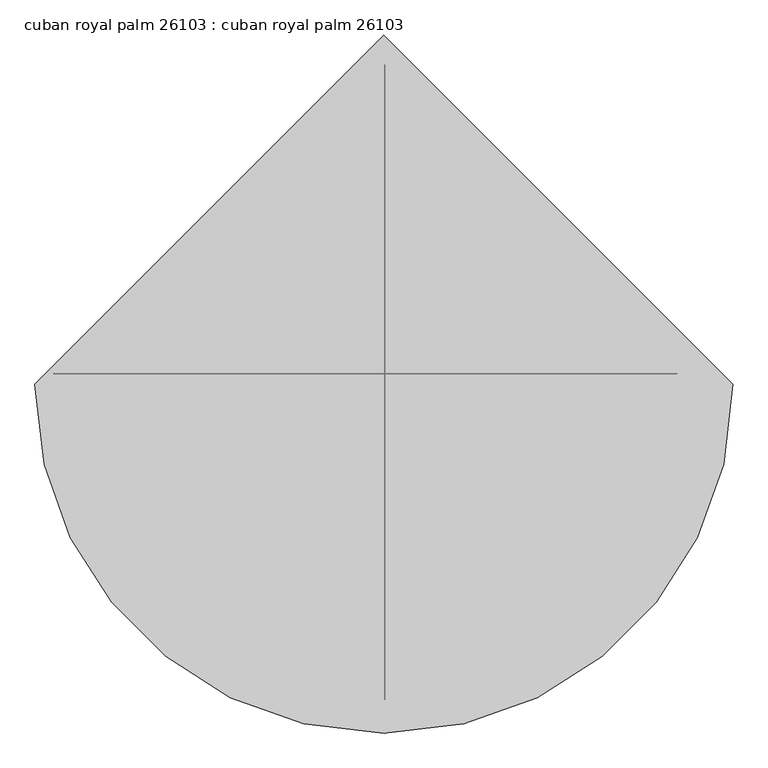
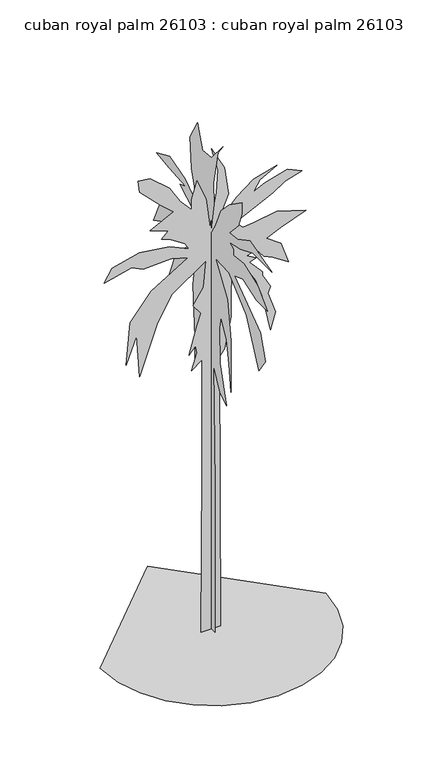
"""IFC4 building model written with IfcOpenShell, lengths in millimetres: proxy geometry, cuban royal palm 26103 : cuban royal palm 26103."""

from ifc_helpers import new_model, si_unit, origin, place, context, project, spatial, triangles, source, transform, mapped, element, save


def cuban_royal_palm_26103_cuban_royal_palm_26103_6f0ceb55(model_context):
    return source(origin(), model_context, "Body", "Tessellation", [
        triangles([(-54.3826135, -0.017491, 0.0009437), (-150.0419681, -0.0174994, 0.0009479), (-130.9099418, -0.0179382, 2494.6483109), (-130.9096875, -0.0182426, 4197.3711227), (-283.9640988, -0.0182154, 4082.5885941), (-207.4377743, -0.0182632, 4331.3053894), (-226.5690375, -0.0182829, 4446.0876274), (-322.2291687, -0.0182582, 4331.3053894), (-207.4375199, -0.0183385, 4752.2081863), (-150.0417137, -0.0183718, 4924.3947693), (-264.8328356, -0.0183942, 5077.4551941), (-111.778179, -0.0184419, 5307.0196701), (-73.5143854, -0.0185154, 5708.7968903), (-570.9431663, -0.0184321, 5364.4237244), (-781.3921303, -0.0183579, 5000.9249817), (-1049.2399527, -0.0182128, 4254.775177), (-1087.5024427, -0.0183274, 4905.2686111), (-1240.5575626, -0.0182489, 4503.4916817), (-1183.1638275, -0.0183643, 5134.8336685), (-877.0535151, -0.0184461, 5517.4841492), (-341.3604137, -0.0185277, 5842.7305756), (-590.0744476, -0.0185305, 5919.260788), (-991.8436014, -0.0185095, 5900.10905), (-1164.030039, -0.0185156, 5976.6392624), (-1565.7991928, -0.018481, 5880.9828918), (-1451.0091064, -0.0185202, 6072.2956329), (-1049.2399527, -0.0185549, 6167.9775833), (-609.2056927, -0.0185639, 6110.5735291), (-322.2291687, -0.0185524, 5976.6392624), (-379.6254836, -0.018567, 6072.2956329), (-609.2056927, -0.0185844, 6225.3560577), (-723.9983225, -0.0185862, 6263.6339539), (-628.3394812, -0.0186075, 6359.2903244), (-896.1847601, -0.0186129, 6454.9461136), (-551.8119212, -0.0186587, 6627.1326965), (-743.1295675, -0.0186811, 6799.3192795), (-1049.2399527, -0.0187225, 7105.4395477), (-1068.3711977, -0.0187524, 7277.6261307), (-896.1847601, -0.0187566, 7258.4743927), (-609.2056927, -0.0187246, 7009.7581787), (-456.1505364, -0.0186868, 6761.0413834), (-283.9640988, -0.0186602, 6569.7286423), (-283.9640988, -0.0186875, 6722.7890671), (-207.4375199, -0.0187388, 6990.6320206), (-73.5143854, -0.0186865, 6665.3850128), (-16.1188494, -0.0186069, 6206.2298996), (79.5405301, -0.0187, 6703.6629089), (98.6725473, -0.0187624, 7048.0354935), (3.0131737, -0.0188232, 7411.5348175), (194.3319064, -0.0187666, 7048.0354935), (251.7277126, -0.0186938, 6627.1326965), (79.5405301, -0.018611, 6206.2298996), (366.5190888, -0.0186818, 6531.476326), (615.2330864, -0.0187268, 6722.7890671), (959.6059616, -0.018759, 6818.4454376), (710.8919277, -0.0187242, 6684.5367508), (615.2330864, -0.0186926, 6531.476326), (787.419524, -0.0187138, 6608.0065384), (1112.6611542, -0.0187452, 6703.6629089), (1323.1125526, -0.0187373, 6608.0065384), (1074.3985914, -0.0187127, 6531.476326), (902.2121538, -0.0186847, 6416.6687988), (347.3878438, -0.0186125, 6148.8258453), (462.1779302, -0.018597, 6034.0433167), (615.2330864, -0.0186071, 6053.1694748), (959.6059616, -0.0186324, 6110.5735291), (1380.5089039, -0.0186269, 5976.6392624), (1017.0023129, -0.018587, 5842.7305756), (806.550769, -0.0185607, 5747.074205), (1017.0023129, -0.0185426, 5594.0143616), (1131.7923992, -0.0184894, 5268.7673538), (902.2121538, -0.0185068, 5421.8277786), (768.288279, -0.0185112, 5479.2062531), (615.2330864, -0.0185387, 5670.544574), (615.2330864, -0.0185284, 5613.1405197), (519.5742451, -0.0185174, 5574.8882034), (653.4956491, -0.0185096, 5498.357991), (557.8367715, -0.0184985, 5460.0800949), (749.1570339, -0.0184693, 5249.6411957), (749.1570339, -0.018459, 5192.2371414), (863.9471203, -0.0184264, 4981.7988235), (825.6846302, -0.0184076, 4886.142453), (940.4747166, -0.0183545, 4560.8957359), (863.9471203, -0.0183067, 4312.1792313), (749.1570339, -0.0184009, 4866.990715), (653.4956491, -0.018448, 5153.9848251), (481.3092115, -0.0184918, 5440.9539368), (309.1227739, -0.0184979, 5517.4841492), (289.9915107, -0.0184287, 5134.8336685), (289.9915107, -0.0183534, 4713.9558701), (194.3319064, -0.0182671, 4254.775177), (117.8043192, -0.0182467, 4159.1188065), (136.9360911, -0.0175052, 0.0009354), (-0.003708, 89.5986644, 0.000495), (-0.0037084, 163.6334895, 0.0005082), (-0.003708, 163.6334895, 1826.7789024), (-0.003706, 145.1250443, 4288.4300995), (-0.0037076, 219.1593699, 4177.3813545), (-0.0037057, 404.2456741, 3788.6856033), (-0.0037071, 404.2456741, 4251.4224747), (-0.0037068, 459.7725537, 5028.7883972), (-0.0037083, 385.7367022, 5565.5410995), (-0.0037091, 533.8058619, 5398.9425476), (-0.0037068, 792.9287807, 4862.190136), (-0.0037064, 1089.0671001, 4492.0362762), (-0.0037084, 1311.1695316, 4140.3737297), (-0.0037071, 1052.0491562, 4843.6988228), (-0.0037074, 885.4710245, 5250.8858871), (-0.0037074, 515.2968899, 5621.065036), (-0.003709, 681.8750216, 5584.0318314), (-0.0037073, 903.9799965, 5565.5410995), (-0.0037076, 1107.5760721, 5602.5487244), (-0.0037076, 1459.2413074, 5417.4588593), (-0.0037087, 1274.1542038, 5824.6462143), (-0.0037067, 1070.5581282, 5824.6462143), (-0.0037071, 996.5223129, 6139.3008453), (-0.0037076, 644.859621, 6065.2600159), (-0.0037089, 422.7546461, 6176.3084702), (-0.0037091, 792.9287807, 6379.9146469), (-0.0037059, 644.859621, 6435.4391647), (-0.0037081, 1052.0491562, 6472.4467896), (-0.0037064, 1385.2054195, 6509.4799942), (-0.0037073, 1052.0491562, 6657.5366547), (-0.0037075, 663.368593, 6546.487619), (-0.0037092, 348.7187945, 6324.3907104), (-0.003707, 496.7904977, 6805.6183136), (-0.0037068, 533.8058619, 7268.3296051), (-0.0037076, 348.7187945, 7601.4755493), (-0.0037068, 311.703394, 7490.427095), (-0.0037069, 219.1593699, 7249.8132935), (-0.0037086, -2.9445681, 7268.3296051), (-0.0037062, -299.0821622, 7619.9924423), (-0.0037078, -169.5227376, 7453.4194702), (-0.0037084, -58.4704863, 6916.6673492), (-0.0037085, -76.9791948, 6602.0121368), (-0.003709, 15.5640629, 6083.7763275), (-0.0037058, -113.9968663, 6287.3575058), (-0.0037085, -243.5573174, 6602.0121368), (-0.0037085, -465.6602757, 6824.1096268), (-0.003709, -780.3075308, 7046.2321152), (-0.003709, -780.3075308, 6879.6341446), (-0.0037083, -687.765287, 6639.0453415), (-0.0037091, -465.6602757, 6398.4315399), (-0.0037063, -669.256315, 6416.9228531), (-0.0037092, -983.9036064, 6583.4958252), (-0.0037074, -1539.164772, 6435.4391647), (-0.0037081, -1057.9394217, 6435.4391647), (-0.0037072, -743.2921303, 6305.8738174), (-0.0037083, -465.6602757, 6250.3492996), (-0.0037076, -558.2050993, 6194.8253632), (-0.003708, -558.2050993, 6102.2932205), (-0.0037077, -835.8344467, 6139.3008453), (-0.0037071, -1187.4996094, 6009.735498), (-0.0037064, -1428.1110855, 5769.1216965), (-0.0037087, -1150.4816654, 5769.1216965), (-0.0037066, -798.8165028, 5880.1701508), (-0.0037081, -595.2230069, 5806.1549011), (-0.0037069, -1243.0264526, 5324.9267166), (-0.0037071, -1372.586713, 4954.7475677), (-0.0037067, -1206.0085814, 4714.1337662), (-0.0037072, -891.36129, 5380.4512344), (-0.0037069, -447.1538472, 5769.1216965), (-0.003706, -113.9968663, 5787.6380081), (-0.0037066, -410.1359396, 5324.9267166), (-0.0037068, -502.6781834, 4751.141391), (-0.0037091, -502.6781834, 3955.2841553), (-0.0037069, -447.1538472, 4362.470929), (-0.003708, -391.6269676, 4695.6171638), (-0.0037083, -243.5573174, 4954.7475677), (-0.0037075, -206.5399003, 4769.6579933), (-0.0037065, -225.0485998, 4232.9058723), (-0.0037092, -391.6269676, 3677.6368584), (-0.0037079, -225.0485998, 3788.6856033), (-0.0037085, -58.4704863, 4103.3405251), (-0.0037063, -95.4881577, 2289.4952808), (-0.0037089, -95.4881577, 0.0004619), (-1653.0963352, -49.1291369, 0.0005424), (-1609.512513, -426.8745255, 0.000473), (-1485.3879673, -773.7746447, 0.0004055), (-1290.6616264, -1079.890044, 0.0003423), (-1035.2724913, -1335.2792519, 0.0002854), (-729.1570919, -1530.0055927, 0.0002372), (-382.2594435, -1654.1301384, 0.0001999), (-4.5121786, -1697.7139606, 0.0001756), (373.234849, -1654.1301384, 0.0001668), (720.1324247, -1530.0055927, 0.0001739), (1026.2478968, -1335.2792519, 0.0001953), (1281.6370319, -1079.890044, 0.0002298), (1476.3633728, -773.7746447, 0.000276), (1600.4879185, -426.8745255, 0.0003326), (1644.0717407, -49.1291369, 0.0003983), (-4.5124832, 1599.4541153, 0.0003027)], [[54, 55, 56], [48, 49, 50], [17, 18, 19], [15, 16, 17], [7, 8, 9], [83, 84, 85], [82, 83, 85], [4, 5, 6], [70, 71, 72], [66, 67, 68], [43, 44, 45], [59, 60, 61], [24, 25, 26], [24, 26, 27], [33, 34, 35], [76, 77, 78], [58, 59, 61], [58, 61, 62], [31, 32, 33], [42, 43, 45], [42, 45, 46], [37, 38, 39], [54, 56, 57], [53, 54, 57], [23, 24, 27], [23, 27, 28], [22, 23, 28], [22, 28, 29], [21, 22, 29], [58, 62, 63], [57, 58, 63], [53, 57, 63], [52, 53, 63], [36, 37, 39], [36, 39, 40], [36, 40, 41], [35, 36, 41], [35, 41, 42], [69, 70, 72], [69, 72, 73], [69, 73, 74], [65, 66, 68], [65, 68, 69], [65, 69, 74], [64, 65, 74], [47, 48, 50], [47, 50, 51], [46, 47, 51], [46, 51, 52], [33, 35, 42], [82, 85, 86], [81, 82, 86], [80, 81, 86], [33, 42, 46], [31, 33, 46], [30, 31, 46], [29, 30, 46], [15, 17, 19], [15, 19, 20], [14, 15, 20], [14, 20, 21], [13, 14, 21], [92, 93, 1], [92, 1, 2], [92, 2, 3], [92, 3, 4], [80, 86, 87], [79, 80, 87], [78, 79, 87], [76, 78, 87], [76, 87, 88], [13, 21, 29], [13, 29, 46], [13, 46, 52], [13, 52, 63], [13, 63, 64], [13, 64, 74], [13, 74, 75], [13, 75, 76], [13, 76, 88], [12, 13, 88], [12, 88, 89], [11, 12, 89], [10, 11, 89], [10, 89, 90], [9, 10, 90], [9, 90, 91], [7, 9, 91], [6, 7, 91], [4, 6, 91], [92, 4, 91], [131, 132, 133], [165, 166, 167], [105, 106, 107], [145, 146, 147], [165, 167, 168], [98, 99, 100], [131, 133, 134], [121, 122, 123], [104, 105, 107], [112, 113, 114], [171, 172, 173], [171, 173, 174], [153, 154, 155], [127, 128, 129], [118, 119, 120], [112, 114, 115], [139, 140, 141], [139, 141, 142], [159, 160, 161], [158, 159, 161], [157, 158, 161], [157, 161, 162], [104, 107, 108], [103, 104, 108], [103, 108, 109], [102, 103, 109], [127, 129, 130], [121, 123, 124], [120, 121, 124], [120, 124, 125], [118, 120, 125], [153, 155, 156], [152, 153, 156], [151, 152, 156], [151, 156, 157], [126, 127, 130], [145, 147, 148], [144, 145, 148], [144, 148, 149], [143, 144, 149], [139, 142, 143], [138, 139, 143], [137, 138, 143], [137, 143, 149], [175, 176, 94], [175, 94, 95], [175, 95, 96], [175, 96, 97], [174, 175, 97], [111, 112, 115], [115, 116, 117], [111, 115, 117], [110, 111, 117], [109, 110, 117], [165, 168, 169], [164, 165, 169], [130, 131, 134], [126, 130, 134], [126, 134, 135], [125, 126, 135], [125, 135, 136], [118, 125, 136], [151, 157, 162], [171, 174, 97], [170, 171, 97], [109, 117, 118], [109, 118, 136], [102, 109, 136], [97, 98, 100], [97, 100, 101], [170, 97, 101], [169, 170, 101], [169, 101, 102], [164, 169, 102], [163, 164, 102], [163, 102, 136], [151, 162, 163], [151, 163, 136], [151, 136, 137], [151, 137, 149], [151, 149, 150], [191, 192, 177], [190, 191, 177], [190, 177, 178], [189, 190, 178], [189, 178, 179], [189, 179, 180], [188, 189, 180], [187, 188, 180], [187, 180, 181], [187, 181, 182], [187, 182, 183], [187, 183, 184], [187, 184, 185], [187, 185, 186]], closed=False),
    ])


if __name__ == "__main__":
    model = new_model("IFC4")
    model_context = context("Model", 3, world=origin())
    ifc_project = project(units=[si_unit("LENGTHUNIT", "METRE", prefix="MILLI")], contexts=[model_context])
    site = spatial("IfcSite", under=ifc_project)
    building = spatial("IfcBuilding", under=site)
    placement = place(None, origin())
    cuban_royal_palm_26103_cuban_royal_palm_26103_shape = cuban_royal_palm_26103_cuban_royal_palm_26103_6f0ceb55(model_context)
    element("IfcBuildingElementProxy", 1, Name="cuban royal palm 26103 : cuban royal palm 26103", ObjectType="cuban royal palm 26103 : cuban royal palm 26103", at=placement, inside=building, context=model_context, shape_type="MappedRepresentation", body=[
        mapped(cuban_royal_palm_26103_cuban_royal_palm_26103_shape, transform((0.0, 0.0, 0.0), x_axis=(1.0, 0.0, 0.0), y_axis=(0.0, 1.0, 0.0), z_axis=(0.0, 0.0, 1.0))),
    ])
    save(model, "model.ifc")

# Revit data of these elements
# Type "cuban royal palm 26103 : cuban royal palm 26103"
#   built-in parameter 1005195 = "RPC-16-FVGV-NKG0-7NHH-C000-ST1L-LVER-AU"
#   Height = 0
